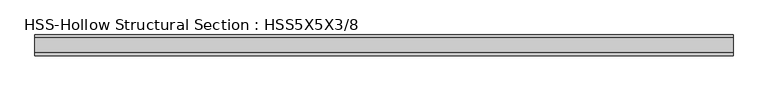
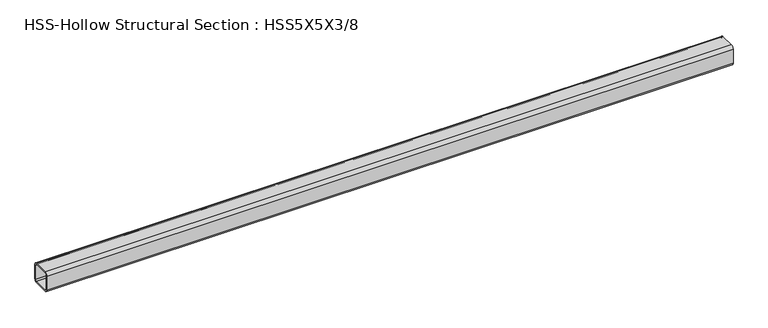
"""IFC4 building model written with IfcOpenShell, lengths in millimetres: beam geometry, HSS-Hollow Structural Section : HSS5X5X3/8."""

from ifc_helpers import new_model, si_unit, point, frame, frame_2d, origin, place, context, project, spatial, polyline, circle_curve, trimmed, segment, composite_curve, outline, extrude, source, transform, mapped, element, save


def hss_hollow_structural_section_hss5x5x3_8_d7d6503a(model_context):
    return source(origin(), model_context, "Body", "SweptSolid", [
        extrude(outline(composite_curve([segment(trimmed(circle_curve(frame_2d((-45.7708, 45.7708)), 17.7292), [point((-63.5, 45.7708))], [point((-45.7708, 63.5))], False, "CARTESIAN"), True, "CONTINUOUS"), segment(polyline([(-45.7708, 63.5), (45.7708, 63.5)]), True, "CONTINUOUS"), segment(trimmed(circle_curve(frame_2d((45.7708, 45.7708)), 17.7292), [point((45.7708, 63.5))], [point((63.5, 45.7708))], False, "CARTESIAN"), True, "CONTINUOUS"), segment(polyline([(63.5, 45.7708), (63.5, -45.7708)]), True, "CONTINUOUS"), segment(trimmed(circle_curve(frame_2d((45.7708, -45.7708)), 17.7292), [point((63.5, -45.7708))], [point((45.7708, -63.5))], False, "CARTESIAN"), True, "CONTINUOUS"), segment(polyline([(45.7708, -63.5), (-45.7708, -63.5)]), True, "CONTINUOUS"), segment(trimmed(circle_curve(frame_2d((-45.7708, -45.7708)), 17.7292), [point((-45.7708, -63.5))], [point((-63.5, -45.7708))], False, "CARTESIAN"), True, "CONTINUOUS"), segment(polyline([(-63.5, -45.7708), (-63.5, 45.7708)]), True, "CONTINUOUS")], self_intersect=False), holes=[composite_curve([segment(polyline([(45.7708, 54.6354), (-45.7708, 54.6354)]), True, "CONTINUOUS"), segment(trimmed(circle_curve(frame_2d((-45.7708, 45.7708)), 8.8646), [point((-45.7708, 54.6354))], [point((-54.6354, 45.7708))], True, "CARTESIAN"), True, "CONTINUOUS"), segment(polyline([(-54.6354, 45.7708), (-54.6354, -45.7708)]), True, "CONTINUOUS"), segment(trimmed(circle_curve(frame_2d((-45.7708, -45.7708)), 8.8646), [point((-54.6354, -45.7708))], [point((-45.7708, -54.6354))], True, "CARTESIAN"), True, "CONTINUOUS"), segment(polyline([(-45.7708, -54.6354), (45.7708, -54.6354)]), True, "CONTINUOUS"), segment(trimmed(circle_curve(frame_2d((45.7708, -45.7708)), 8.8646), [point((45.7708, -54.6354))], [point((54.6354, -45.7708))], True, "CARTESIAN"), True, "CONTINUOUS"), segment(polyline([(54.6354, -45.7708), (54.6354, 45.7708)]), True, "CONTINUOUS"), segment(trimmed(circle_curve(frame_2d((45.7708, 45.7708)), 8.8646), [point((54.6354, 45.7708))], [point((45.7708, 54.6354))], True, "CARTESIAN"), True, "CONTINUOUS")], self_intersect=False)]), frame((-2133.6, 0.0, 0.0), z_axis=(1.0, 0.0, 0.0), x_axis=(0.0, 1.0, 0.0)), (0.0, 0.0, 1.0), 4267.2),
    ])


if __name__ == "__main__":
    model = new_model("IFC4")
    model_context = context("Model", 3, world=origin())
    ifc_project = project(units=[si_unit("LENGTHUNIT", "METRE", prefix="MILLI")], contexts=[model_context])
    site = spatial("IfcSite", under=ifc_project)
    building = spatial("IfcBuilding", under=site)
    placement = place(None, origin())
    hss_hollow_structural_section_hss5x5x3_8_shape = hss_hollow_structural_section_hss5x5x3_8_d7d6503a(model_context)
    element("IfcBeam", 1, ObjectType="HSS-Hollow Structural Section : HSS5X5X3/8", at=placement, inside=building, context=model_context, shape_type="MappedRepresentation", body=[
        mapped(hss_hollow_structural_section_hss5x5x3_8_shape, transform((0.0, 0.0, 0.0), x_axis=(1.0, 0.0, 0.0), y_axis=(0.0, 1.0, 0.0), z_axis=(0.0, 0.0, 1.0))),
    ])
    save(model, "model.ifc")

# Revit data of these elements
# Type "HSS-Hollow Structural Section : HSS5X5X3/8"
#   Assembly Code = "B10"
#   Shape = "Square"
#   W = 22.3
#   Ht = 0' - 5"
#   Length [instance default] = 5' - 0"
#   b = 0' - 5"
#   kr = 0' - 0.698"
#   t = 0' - 0.349"
#   A = 0.0429167 SF
#   Structural Material [instance default] = Steel ASTM A500, Grade B, Rectangular and Square
# Element 1 (IfcBeam, "HSS-Hollow Structural Section : HSS5X5X3/8")
#   Materials on its faces: "Steel ASTM A500, Grade B, Rectangular and Square"
# Materials
#   "Steel ASTM A500, Grade B, Rectangular and Square": class "Metal", colour RGB 199 199 199, transparency 0, Description = "Carbon steel", Cost = 0
